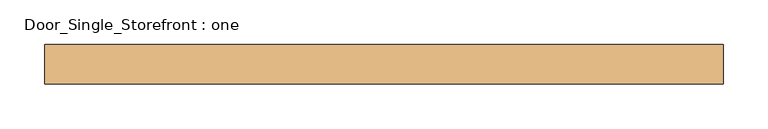
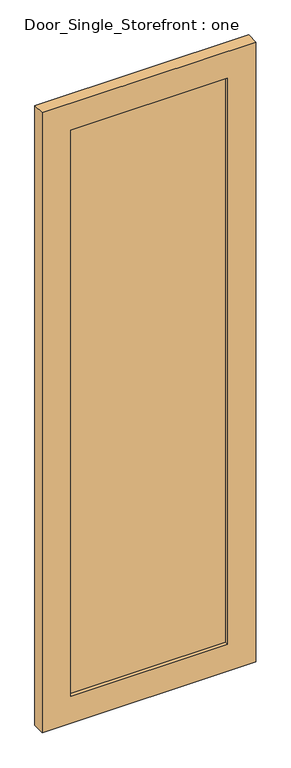
"""IFC4 building model written with IfcOpenShell, lengths in millimetres: door geometry, Door_Single_Storefront : one."""

from ifc_helpers import new_model, si_unit, frame, origin, place, context, project, spatial, polyline, outline, extrude, source, transform, mapped, element, save


def door_single_storefront_one_e33918b4(model_context):
    return source(origin(), model_context, "Body", "SweptSolid", [
        extrude(outline(polyline([(2336.8, -381.0), (0.0, -381.0), (0.0, 381.0), (2336.8, 381.0), (2336.8, -381.0)]), holes=[polyline([(101.6, 279.4), (101.6, -279.4), (2235.2, -279.4), (2235.2, 279.4), (101.6, 279.4)])]), frame((0.0, 6.35, 0.0), z_axis=(0.0, 1.0, 0.0), x_axis=(0.0, 0.0, 1.0)), (0.0, 0.0, 1.0), 44.45),
        extrude(outline(polyline([(279.4, 19.05), (-279.4, 19.05), (-279.4, 38.1), (279.4, 38.1), (279.4, 19.05)])), frame((0.0, 0.0, 101.6), z_axis=(0.0, 0.0, 1.0), x_axis=(1.0, 0.0, 0.0)), (0.0, 0.0, 1.0), 2133.6),
    ])


if __name__ == "__main__":
    model = new_model("IFC4")
    model_context = context("Model", 3, world=origin())
    ifc_project = project(units=[si_unit("LENGTHUNIT", "METRE", prefix="MILLI")], contexts=[model_context])
    site = spatial("IfcSite", under=ifc_project)
    building = spatial("IfcBuilding", under=site)
    placement = place(None, origin())
    door_single_storefront_one_shape = door_single_storefront_one_e33918b4(model_context)
    element("IfcDoor", 1, ObjectType="Door_Single_Storefront : one", at=placement, inside=building, context=model_context, shape_type="MappedRepresentation", body=[
        mapped(door_single_storefront_one_shape, transform((0.0, 0.0, 0.0), x_axis=(1.0, 0.0, 0.0), y_axis=(0.0, 1.0, 0.0), z_axis=(0.0, 0.0, 1.0))),
    ])
    save(model, "model.ifc")

# Revit data of these elements
# Type "Door_Single_Storefront : one"
#   Type Mark = "27"
#   Analytic Construction = "<None>"
#   Stile_Width = 0' - 4"
#   Door_Thickness = 0' - 1 3/4"
#   Door_Offset = 0' - 2"
#   Glass_Material = Glass
#   Frame_Material = Aluminum
#   Function = (empty or 0)
# Element 1 (IfcDoor, "Door_Single_Storefront : one")
#   Materials on its faces: "Aluminum", "Glass"
# Materials
#   "Glass": class "Glass", colour RGB 0 128 192, transparency 0.75, Description = "Soda Lime Glass", Cost = 0
#   "Aluminum": class "Metal", colour RGB 247 247 247, transparency 0, Description = "Aluminum 6061", Cost = 0
